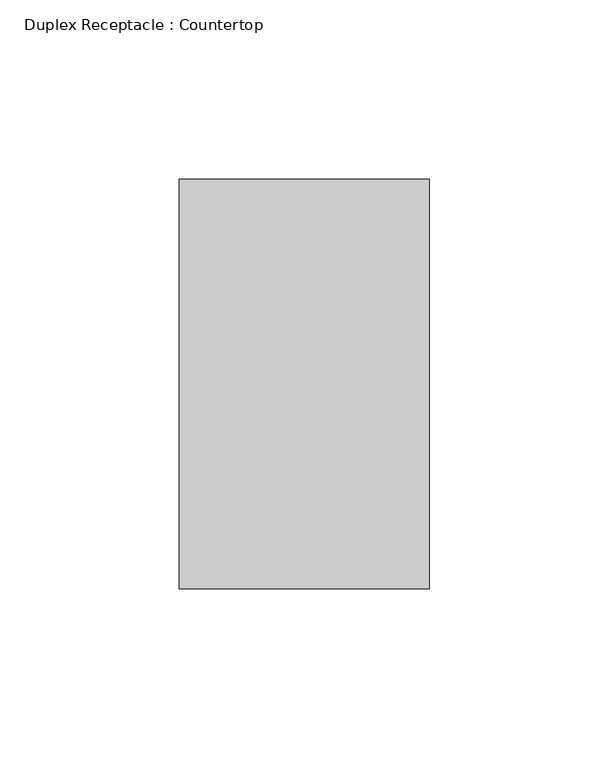
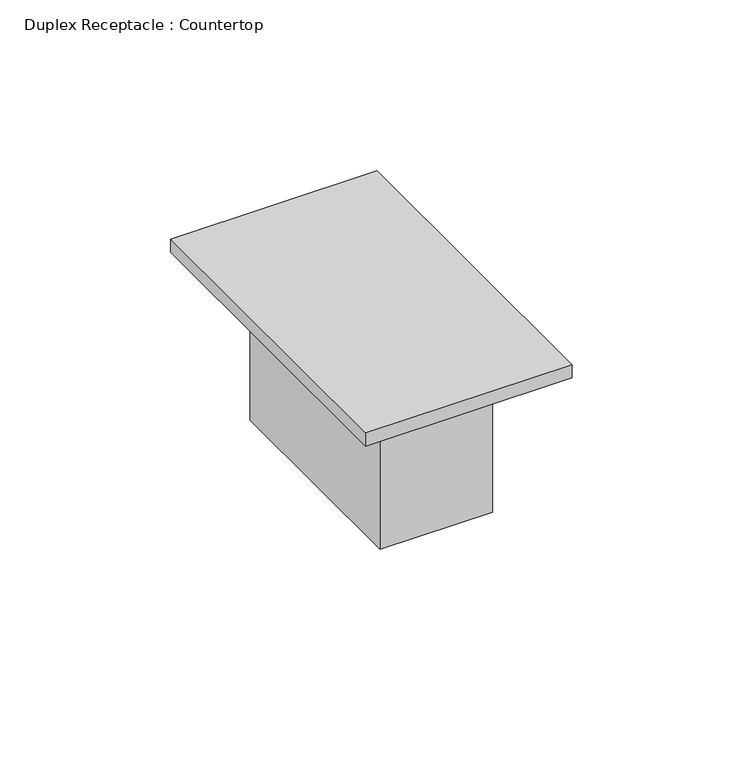
"""IFC4 building model written with IfcOpenShell, lengths in millimetres: proxy geometry, Duplex Receptacle : Countertop."""

from ifc_helpers import new_model, si_unit, frame, origin, origin_with_axes, place, context, project, spatial, polyline, outline, extrude, source, transform, mapped, element, save


def duplex_receptacle_countertop_10251bba(model_context):
    return source(origin(), model_context, "Body", "SweptSolid", [
        extrude(outline(polyline([(19.05, 38.1), (19.05, -38.1), (-19.05, -38.1), (-19.05, 38.1), (19.05, 38.1)])), frame((0.0, 0.0, -53.975), z_axis=(0.0, 0.0, 1.0), x_axis=(1.0, 0.0, 0.0)), (0.0, 0.0, 1.0), 53.975),
        extrude(outline(polyline([(34.925, 57.15), (34.925, -57.15), (-34.925, -57.15), (-34.925, 57.15), (34.925, 57.15)])), origin_with_axes(), (0.0, 0.0, 1.0), 4.7625),
    ])


if __name__ == "__main__":
    model = new_model("IFC4")
    model_context = context("Model", 3, world=origin())
    ifc_project = project(units=[si_unit("LENGTHUNIT", "METRE", prefix="MILLI")], contexts=[model_context])
    site = spatial("IfcSite", under=ifc_project)
    building = spatial("IfcBuilding", under=site)
    placement = place(None, origin())
    duplex_receptacle_countertop_shape = duplex_receptacle_countertop_10251bba(model_context)
    element("IfcBuildingElementProxy", 1, Name="Duplex Receptacle : Countertop", ObjectType="Duplex Receptacle : Countertop", at=placement, inside=building, context=model_context, shape_type="MappedRepresentation", body=[
        mapped(duplex_receptacle_countertop_shape, transform((0.0, 0.0, 0.0), x_axis=(1.0, 0.0, 0.0), y_axis=(0.0, 1.0, 0.0), z_axis=(0.0, 0.0, 1.0))),
    ])
    save(model, "model.ifc")

# Revit data of these elements
# Project information
#   Project Issue Date = "Issue Date"
#   Project Status = "Project Status"
#   Client Name = "Owner"
#   Project Address = "Enter address here"
#   Project Name = "Project Name"
#   Project Number = "Project Number"
#   SR Document GUID = "c3b75027-dcdc-44b1-9c7d-accbc9cf510c"
# Type "Duplex Receptacle : Countertop"
#   Label = "CTR"
#   Switch Voltage = 120 V
#   Load = 180 VA
#   Default Elevation = 1219.2 mm
#   Load Classification = Receptacle
#   Assembly Code = ""
